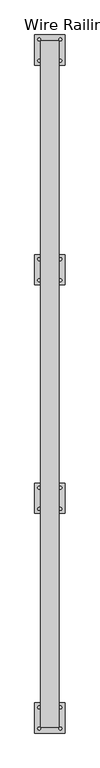
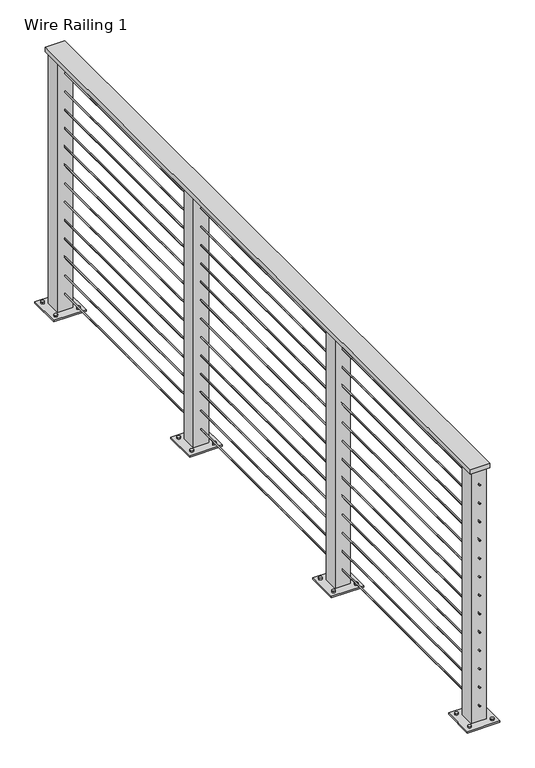
"""IFC4 building model written with IfcOpenShell, lengths in millimetres: railing geometry, Wire Railing 1."""

from ifc_helpers import new_model, si_unit, point, frame, frame_2d, origin, place, context, project, spatial, polyline, circle_curve, trimmed, segment, composite_curve, outline, extrude, source, transform, mapped, element, save


def wire_railing_1_7e8d3eb7(model_context):
    return source(origin(), model_context, "Body", "SweptSolid", [
        extrude(outline(polyline([(-10995.415848, -94.6396465), (-10919.215848, -94.6396465), (-10919.215848, -2977.5396465), (-10995.415848, -2977.5396465), (-10995.415848, -94.6396465)])), frame((0.0, 0.0, 4502.15), z_axis=(0.0, 0.0, 1.0), x_axis=(1.0, 0.0, 0.0)), (0.0, 0.0, 1.0), 19.05),
        extrude(outline(composite_curve([segment(trimmed(circle_curve(frame_2d((4442.61875, -10957.315848)), 2.38125), [point((4442.61875, -10954.934598))], [point((4442.61875, -10959.697098))], False, "CARTESIAN"), True, "CONTINUOUS"), segment(trimmed(circle_curve(frame_2d((4442.61875, -10957.315848)), 2.38125), [point((4442.61875, -10959.697098))], [point((4442.61875, -10954.934598))], False, "CARTESIAN"), True, "CONTINUOUS")], self_intersect=False)), frame((0.0, -2977.5396465, 0.0), z_axis=(0.0, 1.0, 0.0), x_axis=(0.0, 0.0, 1.0)), (0.0, 0.0, 1.0), 2882.9),
        extrude(outline(composite_curve([segment(trimmed(circle_curve(frame_2d((4366.41875, -10957.315848)), 2.38125), [point((4366.41875, -10954.934598))], [point((4366.41875, -10959.697098))], False, "CARTESIAN"), True, "CONTINUOUS"), segment(trimmed(circle_curve(frame_2d((4366.41875, -10957.315848)), 2.38125), [point((4366.41875, -10959.697098))], [point((4366.41875, -10954.934598))], False, "CARTESIAN"), True, "CONTINUOUS")], self_intersect=False)), frame((0.0, -2977.5396465, 0.0), z_axis=(0.0, 1.0, 0.0), x_axis=(0.0, 0.0, 1.0)), (0.0, 0.0, 1.0), 2882.9),
        extrude(outline(composite_curve([segment(trimmed(circle_curve(frame_2d((4290.21875, -10957.315848)), 2.38125), [point((4290.21875, -10954.934598))], [point((4290.21875, -10959.697098))], False, "CARTESIAN"), True, "CONTINUOUS"), segment(trimmed(circle_curve(frame_2d((4290.21875, -10957.315848)), 2.38125), [point((4290.21875, -10959.697098))], [point((4290.21875, -10954.934598))], False, "CARTESIAN"), True, "CONTINUOUS")], self_intersect=False)), frame((0.0, -2977.5396465, 0.0), z_axis=(0.0, 1.0, 0.0), x_axis=(0.0, 0.0, 1.0)), (0.0, 0.0, 1.0), 2882.9),
        extrude(outline(composite_curve([segment(trimmed(circle_curve(frame_2d((4214.01875, -10957.315848)), 2.38125), [point((4214.01875, -10954.934598))], [point((4214.01875, -10959.697098))], False, "CARTESIAN"), True, "CONTINUOUS"), segment(trimmed(circle_curve(frame_2d((4214.01875, -10957.315848)), 2.38125), [point((4214.01875, -10959.697098))], [point((4214.01875, -10954.934598))], False, "CARTESIAN"), True, "CONTINUOUS")], self_intersect=False)), frame((0.0, -2977.5396465, 0.0), z_axis=(0.0, 1.0, 0.0), x_axis=(0.0, 0.0, 1.0)), (0.0, 0.0, 1.0), 2882.9),
        extrude(outline(composite_curve([segment(trimmed(circle_curve(frame_2d((4137.81875, -10957.315848)), 2.38125), [point((4137.81875, -10954.934598))], [point((4137.81875, -10959.697098))], False, "CARTESIAN"), True, "CONTINUOUS"), segment(trimmed(circle_curve(frame_2d((4137.81875, -10957.315848)), 2.38125), [point((4137.81875, -10959.697098))], [point((4137.81875, -10954.934598))], False, "CARTESIAN"), True, "CONTINUOUS")], self_intersect=False)), frame((0.0, -2977.5396465, 0.0), z_axis=(0.0, 1.0, 0.0), x_axis=(0.0, 0.0, 1.0)), (0.0, 0.0, 1.0), 2882.9),
        extrude(outline(composite_curve([segment(trimmed(circle_curve(frame_2d((4061.61875, -10957.315848)), 2.38125), [point((4061.61875, -10954.934598))], [point((4061.61875, -10959.697098))], False, "CARTESIAN"), True, "CONTINUOUS"), segment(trimmed(circle_curve(frame_2d((4061.61875, -10957.315848)), 2.38125), [point((4061.61875, -10959.697098))], [point((4061.61875, -10954.934598))], False, "CARTESIAN"), True, "CONTINUOUS")], self_intersect=False)), frame((0.0, -2977.5396465, 0.0), z_axis=(0.0, 1.0, 0.0), x_axis=(0.0, 0.0, 1.0)), (0.0, 0.0, 1.0), 2882.9),
        extrude(outline(composite_curve([segment(trimmed(circle_curve(frame_2d((3985.41875, -10957.315848)), 2.38125), [point((3985.41875, -10954.934598))], [point((3985.41875, -10959.697098))], False, "CARTESIAN"), True, "CONTINUOUS"), segment(trimmed(circle_curve(frame_2d((3985.41875, -10957.315848)), 2.38125), [point((3985.41875, -10959.697098))], [point((3985.41875, -10954.934598))], False, "CARTESIAN"), True, "CONTINUOUS")], self_intersect=False)), frame((0.0, -2977.5396465, 0.0), z_axis=(0.0, 1.0, 0.0), x_axis=(0.0, 0.0, 1.0)), (0.0, 0.0, 1.0), 2882.9),
        extrude(outline(composite_curve([segment(trimmed(circle_curve(frame_2d((3909.21875, -10957.315848)), 2.38125), [point((3909.21875, -10954.934598))], [point((3909.21875, -10959.697098))], False, "CARTESIAN"), True, "CONTINUOUS"), segment(trimmed(circle_curve(frame_2d((3909.21875, -10957.315848)), 2.38125), [point((3909.21875, -10959.697098))], [point((3909.21875, -10954.934598))], False, "CARTESIAN"), True, "CONTINUOUS")], self_intersect=False)), frame((0.0, -2977.5396465, 0.0), z_axis=(0.0, 1.0, 0.0), x_axis=(0.0, 0.0, 1.0)), (0.0, 0.0, 1.0), 2882.9),
        extrude(outline(composite_curve([segment(trimmed(circle_curve(frame_2d((3833.01875, -10957.315848)), 2.38125), [point((3833.01875, -10954.934598))], [point((3833.01875, -10959.697098))], False, "CARTESIAN"), True, "CONTINUOUS"), segment(trimmed(circle_curve(frame_2d((3833.01875, -10957.315848)), 2.38125), [point((3833.01875, -10959.697098))], [point((3833.01875, -10954.934598))], False, "CARTESIAN"), True, "CONTINUOUS")], self_intersect=False)), frame((0.0, -2977.5396465, 0.0), z_axis=(0.0, 1.0, 0.0), x_axis=(0.0, 0.0, 1.0)), (0.0, 0.0, 1.0), 2882.9),
        extrude(outline(composite_curve([segment(trimmed(circle_curve(frame_2d((3756.81875, -10957.315848)), 2.38125), [point((3756.81875, -10954.934598))], [point((3756.81875, -10959.697098))], False, "CARTESIAN"), True, "CONTINUOUS"), segment(trimmed(circle_curve(frame_2d((3756.81875, -10957.315848)), 2.38125), [point((3756.81875, -10959.697098))], [point((3756.81875, -10954.934598))], False, "CARTESIAN"), True, "CONTINUOUS")], self_intersect=False)), frame((0.0, -2977.5396465, 0.0), z_axis=(0.0, 1.0, 0.0), x_axis=(0.0, 0.0, 1.0)), (0.0, 0.0, 1.0), 2882.9),
        extrude(outline(composite_curve([segment(trimmed(circle_curve(frame_2d((3680.61875, -10957.315848)), 2.38125), [point((3680.61875, -10954.934598))], [point((3680.61875, -10959.697098))], False, "CARTESIAN"), True, "CONTINUOUS"), segment(trimmed(circle_curve(frame_2d((3680.61875, -10957.315848)), 2.38125), [point((3680.61875, -10959.697098))], [point((3680.61875, -10954.934598))], False, "CARTESIAN"), True, "CONTINUOUS")], self_intersect=False)), frame((0.0, -2977.5396465, 0.0), z_axis=(0.0, 1.0, 0.0), x_axis=(0.0, 0.0, 1.0)), (0.0, 0.0, 1.0), 2882.9),
        extrude(outline(composite_curve([segment(trimmed(circle_curve(frame_2d((3604.41875, -10957.315848)), 2.38125), [point((3604.41875, -10954.934598))], [point((3604.41875, -10959.697098))], False, "CARTESIAN"), True, "CONTINUOUS"), segment(trimmed(circle_curve(frame_2d((3604.41875, -10957.315848)), 2.38125), [point((3604.41875, -10959.697098))], [point((3604.41875, -10954.934598))], False, "CARTESIAN"), True, "CONTINUOUS")], self_intersect=False)), frame((0.0, -2977.5396465, 0.0), z_axis=(0.0, 1.0, 0.0), x_axis=(0.0, 0.0, 1.0)), (0.0, 0.0, 1.0), 2882.9),
        extrude(outline(composite_curve([segment(trimmed(circle_curve(frame_2d((3528.21875, -10957.315848)), 2.38125), [point((3528.21875, -10954.934598))], [point((3528.21875, -10959.697098))], False, "CARTESIAN"), True, "CONTINUOUS"), segment(trimmed(circle_curve(frame_2d((3528.21875, -10957.315848)), 2.38125), [point((3528.21875, -10959.697098))], [point((3528.21875, -10954.934598))], False, "CARTESIAN"), True, "CONTINUOUS")], self_intersect=False)), frame((0.0, -2977.5396465, 0.0), z_axis=(0.0, 1.0, 0.0), x_axis=(0.0, 0.0, 1.0)), (0.0, 0.0, 1.0), 2882.9),
        extrude(outline(composite_curve([segment(trimmed(circle_curve(frame_2d((-11001.765848, -1972.1229798)), 6.35), [point((-11008.115848, -1972.1229798))], [point((-10995.415848, -1972.1229798))], False, "CARTESIAN"), True, "CONTINUOUS"), segment(trimmed(circle_curve(frame_2d((-11001.765848, -1972.1229798)), 6.35), [point((-10995.415848, -1972.1229798))], [point((-11008.115848, -1972.1229798))], False, "CARTESIAN"), True, "CONTINUOUS")], self_intersect=False)), frame((0.0, 0.0, 3454.4), z_axis=(0.0, 0.0, 1.0), x_axis=(1.0, 0.0, 0.0)), (0.0, 0.0, 1.0), 12.7),
        extrude(outline(composite_curve([segment(trimmed(circle_curve(frame_2d((-10912.865848, -1972.1229798)), 6.35), [point((-10919.215848, -1972.1229798))], [point((-10906.515848, -1972.1229798))], False, "CARTESIAN"), True, "CONTINUOUS"), segment(trimmed(circle_curve(frame_2d((-10912.865848, -1972.1229798)), 6.35), [point((-10906.515848, -1972.1229798))], [point((-10919.215848, -1972.1229798))], False, "CARTESIAN"), True, "CONTINUOUS")], self_intersect=False)), frame((0.0, 0.0, 3454.4), z_axis=(0.0, 0.0, 1.0), x_axis=(1.0, 0.0, 0.0)), (0.0, 0.0, 1.0), 12.7),
        extrude(outline(composite_curve([segment(trimmed(circle_curve(frame_2d((-11001.765848, -2061.0229798)), 6.35), [point((-11008.115848, -2061.0229798))], [point((-10995.415848, -2061.0229798))], False, "CARTESIAN"), True, "CONTINUOUS"), segment(trimmed(circle_curve(frame_2d((-11001.765848, -2061.0229798)), 6.35), [point((-10995.415848, -2061.0229798))], [point((-11008.115848, -2061.0229798))], False, "CARTESIAN"), True, "CONTINUOUS")], self_intersect=False)), frame((0.0, 0.0, 3454.4), z_axis=(0.0, 0.0, 1.0), x_axis=(1.0, 0.0, 0.0)), (0.0, 0.0, 1.0), 12.7),
        extrude(outline(composite_curve([segment(trimmed(circle_curve(frame_2d((-10912.865848, -2061.0229798)), 6.35), [point((-10919.215848, -2061.0229798))], [point((-10906.515848, -2061.0229798))], False, "CARTESIAN"), True, "CONTINUOUS"), segment(trimmed(circle_curve(frame_2d((-10912.865848, -2061.0229798)), 6.35), [point((-10906.515848, -2061.0229798))], [point((-10919.215848, -2061.0229798))], False, "CARTESIAN"), True, "CONTINUOUS")], self_intersect=False)), frame((0.0, 0.0, 3454.4), z_axis=(0.0, 0.0, 1.0), x_axis=(1.0, 0.0, 0.0)), (0.0, 0.0, 1.0), 12.7),
        extrude(outline(polyline([(-10893.815848, -1953.0729798), (-10893.815848, -2080.0729798), (-11020.815848, -2080.0729798), (-11020.815848, -1953.0729798), (-10893.815848, -1953.0729798)])), frame((0.0, 0.0, 3454.4), z_axis=(0.0, 0.0, 1.0), x_axis=(1.0, 0.0, 0.0)), (0.0, 0.0, 1.0), 6.35),
        extrude(outline(polyline([(-10927.153348, -1986.4104798), (-10927.153348, -2046.7354798), (-10987.478348, -2046.7354798), (-10987.478348, -1986.4104798), (-10927.153348, -1986.4104798)]), holes=[polyline([(-10933.503348, -1992.7604798), (-10981.128348, -1992.7604798), (-10981.128348, -2040.3854798), (-10933.503348, -2040.3854798), (-10933.503348, -1992.7604798)])]), frame((0.0, 0.0, 3454.4), z_axis=(0.0, 0.0, 1.0), x_axis=(1.0, 0.0, 0.0)), (0.0, 0.0, 1.0), 1047.75),
        extrude(outline(composite_curve([segment(trimmed(circle_curve(frame_2d((-11001.765848, -1011.1563132)), 6.35), [point((-11008.115848, -1011.1563132))], [point((-10995.415848, -1011.1563132))], False, "CARTESIAN"), True, "CONTINUOUS"), segment(trimmed(circle_curve(frame_2d((-11001.765848, -1011.1563132)), 6.35), [point((-10995.415848, -1011.1563132))], [point((-11008.115848, -1011.1563132))], False, "CARTESIAN"), True, "CONTINUOUS")], self_intersect=False)), frame((0.0, 0.0, 3454.4), z_axis=(0.0, 0.0, 1.0), x_axis=(1.0, 0.0, 0.0)), (0.0, 0.0, 1.0), 12.7),
        extrude(outline(composite_curve([segment(trimmed(circle_curve(frame_2d((-10912.865848, -1011.1563132)), 6.35), [point((-10919.215848, -1011.1563132))], [point((-10906.515848, -1011.1563132))], False, "CARTESIAN"), True, "CONTINUOUS"), segment(trimmed(circle_curve(frame_2d((-10912.865848, -1011.1563132)), 6.35), [point((-10906.515848, -1011.1563132))], [point((-10919.215848, -1011.1563132))], False, "CARTESIAN"), True, "CONTINUOUS")], self_intersect=False)), frame((0.0, 0.0, 3454.4), z_axis=(0.0, 0.0, 1.0), x_axis=(1.0, 0.0, 0.0)), (0.0, 0.0, 1.0), 12.7),
        extrude(outline(composite_curve([segment(trimmed(circle_curve(frame_2d((-11001.765848, -1100.0563132)), 6.35), [point((-11008.115848, -1100.0563132))], [point((-10995.415848, -1100.0563132))], False, "CARTESIAN"), True, "CONTINUOUS"), segment(trimmed(circle_curve(frame_2d((-11001.765848, -1100.0563132)), 6.35), [point((-10995.415848, -1100.0563132))], [point((-11008.115848, -1100.0563132))], False, "CARTESIAN"), True, "CONTINUOUS")], self_intersect=False)), frame((0.0, 0.0, 3454.4), z_axis=(0.0, 0.0, 1.0), x_axis=(1.0, 0.0, 0.0)), (0.0, 0.0, 1.0), 12.7),
        extrude(outline(composite_curve([segment(trimmed(circle_curve(frame_2d((-10912.865848, -1100.0563132)), 6.35), [point((-10919.215848, -1100.0563132))], [point((-10906.515848, -1100.0563132))], False, "CARTESIAN"), True, "CONTINUOUS"), segment(trimmed(circle_curve(frame_2d((-10912.865848, -1100.0563132)), 6.35), [point((-10906.515848, -1100.0563132))], [point((-10919.215848, -1100.0563132))], False, "CARTESIAN"), True, "CONTINUOUS")], self_intersect=False)), frame((0.0, 0.0, 3454.4), z_axis=(0.0, 0.0, 1.0), x_axis=(1.0, 0.0, 0.0)), (0.0, 0.0, 1.0), 12.7),
        extrude(outline(polyline([(-10893.815848, -992.1063132), (-10893.815848, -1119.1063132), (-11020.815848, -1119.1063132), (-11020.815848, -992.1063132), (-10893.815848, -992.1063132)])), frame((0.0, 0.0, 3454.4), z_axis=(0.0, 0.0, 1.0), x_axis=(1.0, 0.0, 0.0)), (0.0, 0.0, 1.0), 6.35),
        extrude(outline(polyline([(-10927.153348, -1025.4438132), (-10927.153348, -1085.7688132), (-10987.478348, -1085.7688132), (-10987.478348, -1025.4438132), (-10927.153348, -1025.4438132)]), holes=[polyline([(-10933.503348, -1031.7938132), (-10981.128348, -1031.7938132), (-10981.128348, -1079.4188132), (-10933.503348, -1079.4188132), (-10933.503348, -1031.7938132)])]), frame((0.0, 0.0, 3454.4), z_axis=(0.0, 0.0, 1.0), x_axis=(1.0, 0.0, 0.0)), (0.0, 0.0, 1.0), 1047.75),
        extrude(outline(composite_curve([segment(trimmed(circle_curve(frame_2d((-11001.765848, -2894.9896465)), 6.35), [point((-11008.115848, -2894.9896465))], [point((-10995.415848, -2894.9896465))], False, "CARTESIAN"), True, "CONTINUOUS"), segment(trimmed(circle_curve(frame_2d((-11001.765848, -2894.9896465)), 6.35), [point((-10995.415848, -2894.9896465))], [point((-11008.115848, -2894.9896465))], False, "CARTESIAN"), True, "CONTINUOUS")], self_intersect=False)), frame((0.0, 0.0, 3454.4), z_axis=(0.0, 0.0, 1.0), x_axis=(1.0, 0.0, 0.0)), (0.0, 0.0, 1.0), 12.7),
        extrude(outline(composite_curve([segment(trimmed(circle_curve(frame_2d((-10912.865848, -2894.9896465)), 6.35), [point((-10919.215848, -2894.9896465))], [point((-10906.515848, -2894.9896465))], False, "CARTESIAN"), True, "CONTINUOUS"), segment(trimmed(circle_curve(frame_2d((-10912.865848, -2894.9896465)), 6.35), [point((-10906.515848, -2894.9896465))], [point((-10919.215848, -2894.9896465))], False, "CARTESIAN"), True, "CONTINUOUS")], self_intersect=False)), frame((0.0, 0.0, 3454.4), z_axis=(0.0, 0.0, 1.0), x_axis=(1.0, 0.0, 0.0)), (0.0, 0.0, 1.0), 12.7),
        extrude(outline(composite_curve([segment(trimmed(circle_curve(frame_2d((-11001.765848, -2983.8896465)), 6.35), [point((-11008.115848, -2983.8896465))], [point((-10995.415848, -2983.8896465))], False, "CARTESIAN"), True, "CONTINUOUS"), segment(trimmed(circle_curve(frame_2d((-11001.765848, -2983.8896465)), 6.35), [point((-10995.415848, -2983.8896465))], [point((-11008.115848, -2983.8896465))], False, "CARTESIAN"), True, "CONTINUOUS")], self_intersect=False)), frame((0.0, 0.0, 3454.4), z_axis=(0.0, 0.0, 1.0), x_axis=(1.0, 0.0, 0.0)), (0.0, 0.0, 1.0), 12.7),
        extrude(outline(composite_curve([segment(trimmed(circle_curve(frame_2d((-10912.865848, -2983.8896465)), 6.35), [point((-10919.215848, -2983.8896465))], [point((-10906.515848, -2983.8896465))], False, "CARTESIAN"), True, "CONTINUOUS"), segment(trimmed(circle_curve(frame_2d((-10912.865848, -2983.8896465)), 6.35), [point((-10906.515848, -2983.8896465))], [point((-10919.215848, -2983.8896465))], False, "CARTESIAN"), True, "CONTINUOUS")], self_intersect=False)), frame((0.0, 0.0, 3454.4), z_axis=(0.0, 0.0, 1.0), x_axis=(1.0, 0.0, 0.0)), (0.0, 0.0, 1.0), 12.7),
        extrude(outline(polyline([(-10893.815848, -2875.9396465), (-10893.815848, -3002.9396465), (-11020.815848, -3002.9396465), (-11020.815848, -2875.9396465), (-10893.815848, -2875.9396465)])), frame((0.0, 0.0, 3454.4), z_axis=(0.0, 0.0, 1.0), x_axis=(1.0, 0.0, 0.0)), (0.0, 0.0, 1.0), 6.35),
        extrude(outline(polyline([(-10927.153348, -2909.2771465), (-10927.153348, -2969.6021465), (-10987.478348, -2969.6021465), (-10987.478348, -2909.2771465), (-10927.153348, -2909.2771465)]), holes=[polyline([(-10933.503348, -2915.6271465), (-10981.128348, -2915.6271465), (-10981.128348, -2963.2521465), (-10933.503348, -2963.2521465), (-10933.503348, -2915.6271465)])]), frame((0.0, 0.0, 3454.4), z_axis=(0.0, 0.0, 1.0), x_axis=(1.0, 0.0, 0.0)), (0.0, 0.0, 1.0), 1047.75),
        extrude(outline(composite_curve([segment(trimmed(circle_curve(frame_2d((-11001.765848, -88.2896465)), 6.35), [point((-11008.115848, -88.2896465))], [point((-10995.415848, -88.2896465))], False, "CARTESIAN"), True, "CONTINUOUS"), segment(trimmed(circle_curve(frame_2d((-11001.765848, -88.2896465)), 6.35), [point((-10995.415848, -88.2896465))], [point((-11008.115848, -88.2896465))], False, "CARTESIAN"), True, "CONTINUOUS")], self_intersect=False)), frame((0.0, 0.0, 3454.4), z_axis=(0.0, 0.0, 1.0), x_axis=(1.0, 0.0, 0.0)), (0.0, 0.0, 1.0), 12.7),
        extrude(outline(composite_curve([segment(trimmed(circle_curve(frame_2d((-10912.865848, -88.2896465)), 6.35), [point((-10919.215848, -88.2896465))], [point((-10906.515848, -88.2896465))], False, "CARTESIAN"), True, "CONTINUOUS"), segment(trimmed(circle_curve(frame_2d((-10912.865848, -88.2896465)), 6.35), [point((-10906.515848, -88.2896465))], [point((-10919.215848, -88.2896465))], False, "CARTESIAN"), True, "CONTINUOUS")], self_intersect=False)), frame((0.0, 0.0, 3454.4), z_axis=(0.0, 0.0, 1.0), x_axis=(1.0, 0.0, 0.0)), (0.0, 0.0, 1.0), 12.7),
        extrude(outline(composite_curve([segment(trimmed(circle_curve(frame_2d((-11001.765848, -177.1896465)), 6.35), [point((-11008.115848, -177.1896465))], [point((-10995.415848, -177.1896465))], False, "CARTESIAN"), True, "CONTINUOUS"), segment(trimmed(circle_curve(frame_2d((-11001.765848, -177.1896465)), 6.35), [point((-10995.415848, -177.1896465))], [point((-11008.115848, -177.1896465))], False, "CARTESIAN"), True, "CONTINUOUS")], self_intersect=False)), frame((0.0, 0.0, 3454.4), z_axis=(0.0, 0.0, 1.0), x_axis=(1.0, 0.0, 0.0)), (0.0, 0.0, 1.0), 12.7),
        extrude(outline(composite_curve([segment(trimmed(circle_curve(frame_2d((-10912.865848, -177.1896465)), 6.35), [point((-10919.215848, -177.1896465))], [point((-10906.515848, -177.1896465))], False, "CARTESIAN"), True, "CONTINUOUS"), segment(trimmed(circle_curve(frame_2d((-10912.865848, -177.1896465)), 6.35), [point((-10906.515848, -177.1896465))], [point((-10919.215848, -177.1896465))], False, "CARTESIAN"), True, "CONTINUOUS")], self_intersect=False)), frame((0.0, 0.0, 3454.4), z_axis=(0.0, 0.0, 1.0), x_axis=(1.0, 0.0, 0.0)), (0.0, 0.0, 1.0), 12.7),
        extrude(outline(polyline([(-10893.815848, -69.2396465), (-10893.815848, -196.2396465), (-11020.815848, -196.2396465), (-11020.815848, -69.2396465), (-10893.815848, -69.2396465)])), frame((0.0, 0.0, 3454.4), z_axis=(0.0, 0.0, 1.0), x_axis=(1.0, 0.0, 0.0)), (0.0, 0.0, 1.0), 6.35),
        extrude(outline(polyline([(-10927.153348, -102.5771465), (-10927.153348, -162.9021465), (-10987.478348, -162.9021465), (-10987.478348, -102.5771465), (-10927.153348, -102.5771465)]), holes=[polyline([(-10933.503348, -108.9271465), (-10981.128348, -108.9271465), (-10981.128348, -156.5521465), (-10933.503348, -156.5521465), (-10933.503348, -108.9271465)])]), frame((0.0, 0.0, 3454.4), z_axis=(0.0, 0.0, 1.0), x_axis=(1.0, 0.0, 0.0)), (0.0, 0.0, 1.0), 1047.75),
    ])


if __name__ == "__main__":
    model = new_model("IFC4")
    model_context = context("Model", 3, world=origin())
    ifc_project = project(units=[si_unit("LENGTHUNIT", "METRE", prefix="MILLI")], contexts=[model_context])
    site = spatial("IfcSite", under=ifc_project)
    building = spatial("IfcBuilding", under=site)
    placement = place(None, origin())
    wire_railing_1_shape = wire_railing_1_7e8d3eb7(model_context)
    element("IfcRailing", 1, ObjectType="Wire Railing 1", at=placement, inside=building, context=model_context, shape_type="MappedRepresentation", body=[
        mapped(wire_railing_1_shape, transform((0.0, 0.0, 0.0), x_axis=(1.0, 0.0, 0.0), y_axis=(0.0, 1.0, 0.0), z_axis=(0.0, 0.0, 1.0))),
    ])
    save(model, "model.ifc")

# Revit data of these elements
# Element 1 (IfcRailing, "Wire Railing 1")
#   Materials on its faces: "Metal - Kawneer - Aluminum"
# Materials
#   "Metal - Kawneer - Aluminum": class "Metal", colour RGB 244 244 244, transparency 0, Manufacturer = "Kawneer", URL = "http://www.kawneer.com/kawneer/north_america/en/home.asp", Cost = 0
